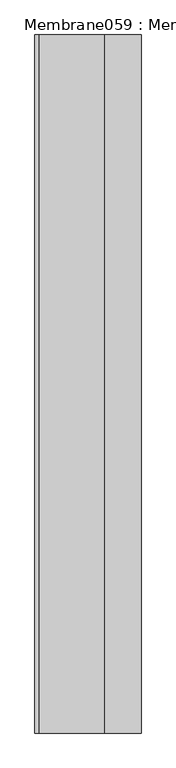
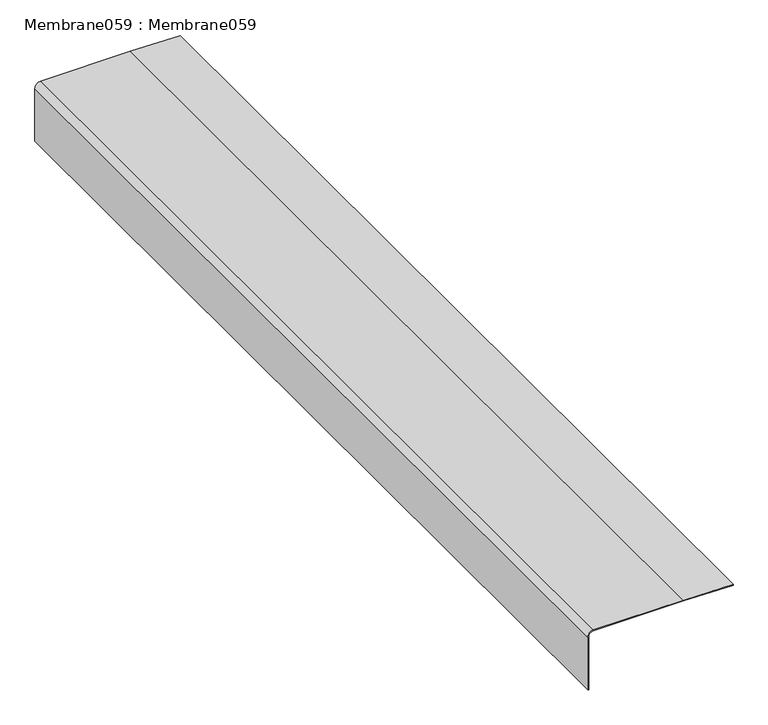
"""IFC4 building model written with IfcOpenShell, lengths in millimetres: proxy geometry, Membrane059 : Membrane059."""

from ifc_helpers import new_model, si_unit, point, frame, frame_2d, origin, place, context, project, spatial, polyline, circle_curve, trimmed, segment, composite_curve, outline, extrude, source, transform, mapped, element, save


def membrane059_membrane059_305fa67c(model_context):
    return source(origin(), model_context, "Body", "SweptSolid", [
        extrude(outline(composite_curve([segment(trimmed(circle_curve(frame_2d((40233.3001163, -4991.7403478)), 10.0), [point((40233.3001163, -5001.7403478))], [point((40243.3001163, -4991.7403478))], True, "CARTESIAN"), True, "CONTINUOUS"), segment(polyline([(40243.3001163, -4991.7403478), (40243.3001163, -4804.1710546), (40241.7972226, -4699.8063764), (40243.79743, -4699.8063764), (40245.3001163, -4804.1566552), (40245.3001163, -4991.7403478)]), True, "CONTINUOUS"), segment(trimmed(circle_curve(frame_2d((40233.3001163, -4991.7403478)), 12.0), [point((40245.3001163, -4991.7403478))], [point((40233.3001163, -5003.7403478))], False, "CARTESIAN"), True, "CONTINUOUS"), segment(polyline([(40233.3001163, -5003.7403478), (40116.5801181, -5003.7403478), (40116.5801181, -5001.7403478), (40233.3001163, -5001.7403478)]), True, "CONTINUOUS")], self_intersect=False)), frame((0.0, -1052.8906574, 0.0), z_axis=(0.0, 1.0, 0.0), x_axis=(0.0, 0.0, 1.0)), (0.0, 0.0, 1.0), 2000.0),
    ])


if __name__ == "__main__":
    model = new_model("IFC4")
    model_context = context("Model", 3, world=origin())
    ifc_project = project(units=[si_unit("LENGTHUNIT", "METRE", prefix="MILLI")], contexts=[model_context])
    site = spatial("IfcSite", under=ifc_project)
    building = spatial("IfcBuilding", under=site)
    placement = place(None, origin())
    membrane059_membrane059_shape = membrane059_membrane059_305fa67c(model_context)
    element("IfcBuildingElementProxy", 1, Name="Membrane059 : Membrane059", ObjectType="Membrane059 : Membrane059", at=placement, inside=building, context=model_context, shape_type="MappedRepresentation", body=[
        mapped(membrane059_membrane059_shape, transform((0.0, 0.0, 0.0), x_axis=(1.0, 0.0, 0.0), y_axis=(0.0, 1.0, 0.0), z_axis=(0.0, 0.0, 1.0))),
    ])
    save(model, "model.ifc")

# Revit data of these elements
# Type "Membrane059 : Membrane059"
#   NameOverride = "Membrane059"
# Element 1 (IfcBuildingElementProxy, "Membrane059 : Membrane059")
#   Materials on its faces: "THREE PLY BUILT UP ROOF MEMBRANE"
# Materials
#   "THREE PLY BUILT UP ROOF MEMBRANE": class "Unassigned", colour RGB 63 63 63, transparency 0
